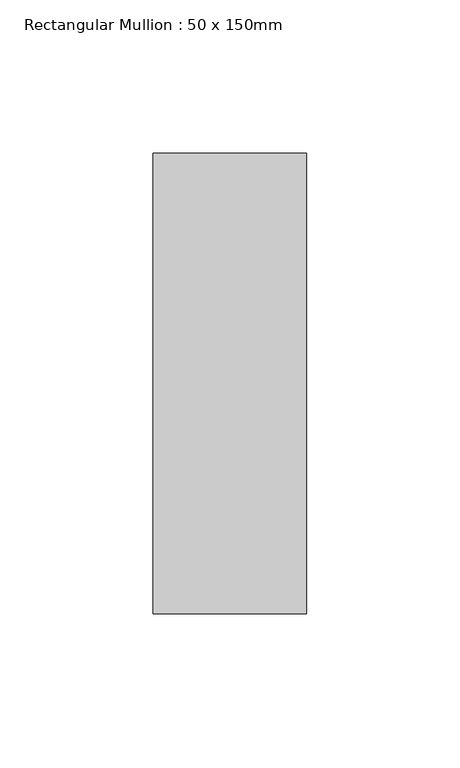
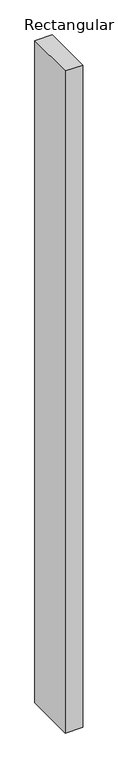
"""IFC4 building model written with IfcOpenShell, lengths in millimetres: member geometry, Rectangular Mullion : 50 x 150mm."""

import ifcopenshell
import ifcopenshell.guid

model = None  # the IFC model being written
_history = None  # IfcOwnerHistory: only IFC2X3 demands one
_inside = {}  # id of a spatial element -> (the spatial element, [elements in it])
_under = {}  # id of a project, library or spatial element -> (it, [spatial elements below it])
_declared = {}  # id of a project -> (the project, [libraries it declares])
_typed = {}  # id of a type object -> (the type object, [elements of that type])
_made_of = {}  # id of a material, layer set ... -> (it, [elements and type objects made of it])


def new_model(schema):
    """Start an empty IFC model of exactly this schema.

    Asked for "IFC4X3", IfcOpenShell would pick the latest addendum, in which some entities
    have other attributes; the version numbers below select the first issue.
    IFC2X3 requires an IfcOwnerHistory on every rooted entity: one is made here for all.
    """
    global model, _history
    if schema == "IFC4X3":
        model = ifcopenshell.file(schema_version=(4, 3, 0, 0))
    else:
        model = ifcopenshell.file(schema=schema)
    _inside.clear()
    _under.clear()
    _declared.clear()
    _typed.clear()
    _made_of.clear()
    _history = None
    if model.schema == "IFC2X3":
        org = make("IfcOrganization", Name="unknown")
        user = make(
            "IfcPersonAndOrganization",
            ThePerson=make("IfcPerson", FamilyName="unknown"),
            TheOrganization=org,
        )
        app = make(
            "IfcApplication",
            ApplicationDeveloper=org,
            Version="unknown",
            ApplicationFullName="unknown",
            ApplicationIdentifier="unknown",
        )
        _history = make(
            "IfcOwnerHistory",
            OwningUser=user,
            OwningApplication=app,
            ChangeAction="ADDED",
            CreationDate=0,
        )
    return model


def make(cls, **values):
    """One entity of the class cls with the attributes given. An attribute that is None is left unset."""
    return model.create_entity(
        cls, **{name: value for name, value in values.items() if value is not None}
    )


def rooted(cls, **values):
    """An entity with a GlobalId (a new one), such as an element, a storey or a relation."""
    return make(cls, GlobalId=ifcopenshell.guid.new(), OwnerHistory=_history, **values)


def si_unit(unit_type, name, prefix=None):
    """IfcSIUnit, for example si_unit("LENGTHUNIT", "METRE", prefix="MILLI")."""
    return make("IfcSIUnit", UnitType=unit_type, Prefix=prefix, Name=name)


def assignment(units):
    """IfcUnitAssignment: the units of a project."""
    return None if units is None else make("IfcUnitAssignment", Units=units)


def point(xyz):
    """IfcCartesianPoint."""
    return None if xyz is None else make("IfcCartesianPoint", Coordinates=xyz)


def direction(xyz):
    """IfcDirection."""
    return None if xyz is None else make("IfcDirection", DirectionRatios=xyz)


def frame(location, z_axis=None, x_axis=None):
    """IfcAxis2Placement3D, a coordinate frame: its origin and axes. An axis left out is left unset."""
    return make(
        "IfcAxis2Placement3D",
        Location=point(location),
        Axis=direction(z_axis),
        RefDirection=direction(x_axis),
    )


def origin():
    """The frame at (0, 0, 0) with its axes left unset."""
    return frame((0.0, 0.0, 0.0))


def place(relative_to, where):
    """IfcLocalPlacement: puts the frame where relative to a parent placement (None: the world)."""
    return make(
        "IfcLocalPlacement", PlacementRelTo=relative_to, RelativePlacement=where
    )


def context(
    kind, dimensions, precision=None, world=None, true_north=None, identifier=None
):
    """IfcGeometricRepresentationContext, for example the 3D "Model" context."""
    return make(
        "IfcGeometricRepresentationContext",
        ContextIdentifier=identifier,
        ContextType=kind,
        CoordinateSpaceDimension=dimensions,
        Precision=precision,
        WorldCoordinateSystem=world,
        TrueNorth=true_north,
    )


def project(units=None, contexts=None):
    """IfcProject with its units and contexts."""
    return rooted(
        "IfcProject",
        Name="project",
        RepresentationContexts=contexts,
        UnitsInContext=assignment(units),
    )


def spatial(cls, under=None, at=None, **own):
    """A site, building, storey or space (cls), placed at a placement, below another one or the project."""
    s = rooted(cls, ObjectPlacement=at, **own)
    if under is not None:
        _under.setdefault(under.id(), (under, []))[1].append(s)
    return s


def polyline(points):
    """IfcPolyline through the points."""
    return make("IfcPolyline", Points=[point(p) for p in points])


def outline(outer, holes=None, kind="AREA"):
    """IfcArbitraryClosedProfileDef: a profile drawn as a closed curve; with holes, ...WithVoids."""
    if holes is None:
        return make("IfcArbitraryClosedProfileDef", ProfileType=kind, OuterCurve=outer)
    return make(
        "IfcArbitraryProfileDefWithVoids",
        ProfileType=kind,
        OuterCurve=outer,
        InnerCurves=holes,
    )


def extrude(swept, where, along, depth):
    """IfcExtrudedAreaSolid: the profile swept, set in the frame where, extruded along a direction by depth."""
    return make(
        "IfcExtrudedAreaSolid",
        SweptArea=swept,
        Position=where,
        ExtrudedDirection=direction(along),
        Depth=depth,
    )


def shape(context_of_items, identifier, shape_type, items):
    """IfcShapeRepresentation: the items that make up one representation, for example the "Body"."""
    return make(
        "IfcShapeRepresentation",
        ContextOfItems=context_of_items,
        RepresentationIdentifier=identifier,
        RepresentationType=shape_type,
        Items=items,
    )


def source(mapping_origin, context_of_items, identifier, shape_type, items):
    """IfcRepresentationMap: a shape defined once, which mapped items show again and again."""
    return make(
        "IfcRepresentationMap",
        MappingOrigin=mapping_origin,
        MappedRepresentation=shape(context_of_items, identifier, shape_type, items),
    )


def transform(
    local_origin,
    x_axis=None,
    y_axis=None,
    z_axis=None,
    scale=None,
    scale2=None,
    scale3=None,
    uniform=True,
):
    """IfcCartesianTransformationOperator3D, or its non-uniform kind. x_axis, y_axis, z_axis: its Axis1, 2, 3."""
    if uniform:
        return make(
            "IfcCartesianTransformationOperator3D",
            Axis1=direction(x_axis),
            Axis2=direction(y_axis),
            LocalOrigin=point(local_origin),
            Scale=scale,
            Axis3=direction(z_axis),
        )
    return make(
        "IfcCartesianTransformationOperator3DnonUniform",
        Axis1=direction(x_axis),
        Axis2=direction(y_axis),
        LocalOrigin=point(local_origin),
        Scale=scale,
        Axis3=direction(z_axis),
        Scale2=scale2,
        Scale3=scale3,
    )


def mapped(mapping_source, mapping_target):
    """IfcMappedItem: shows the shape of a source again, moved by a transform."""
    return make(
        "IfcMappedItem", MappingSource=mapping_source, MappingTarget=mapping_target
    )


def made_of(thing, what):
    """Note that an element or type object is made of a material, layer set ...; save() writes the relation."""
    if what is not None:
        _made_of.setdefault(what.id(), (what, []))[1].append(thing)
    return thing


def element(
    cls,
    number,
    at=None,
    inside=None,
    cuts=None,
    type_object=None,
    material=None,
    context=None,
    identifier="Body",
    shape_type=None,
    held_by="IfcProductDefinitionShape",
    body=None,
    shapes=None,
    **own,
):
    """One element of the class cls, such as IfcWall. Its Tag is "e" and its number.

    at: its placement. inside: the storey or other place that contains it. cuts: it is an
    opening in that element (IfcRelVoidsElement). A single representation is given by context,
    identifier, shape_type and body (its items); several are given by shapes. held_by: the class
    of the entity that holds the representations. save() writes the other relations.
    """
    e = rooted(cls, Tag="e%d" % number, ObjectPlacement=at, **own)
    if body is not None:
        shapes = [shape(context, identifier, shape_type, body)]
    if shapes is not None:
        e.Representation = make(held_by, Representations=shapes)
    if inside is not None:
        _inside.setdefault(inside.id(), (inside, []))[1].append(e)
    if cuts is not None:
        rooted(
            "IfcRelVoidsElement", RelatingBuildingElement=cuts, RelatedOpeningElement=e
        )
    if type_object is not None:
        _typed.setdefault(type_object.id(), (type_object, []))[1].append(e)
    return made_of(e, material)


def aggregate(whole, parts):
    """IfcRelAggregates: a whole, such as a stair, and the parts it consists of."""
    return rooted("IfcRelAggregates", RelatingObject=whole, RelatedObjects=parts)


def save(model, path):
    """Write the relations noted so far, then the file.

    IfcRelAggregates (storeys below a building ...), IfcRelContainedInSpatialStructure (elements
    in a storey), IfcRelDefinesByType, IfcRelAssociatesMaterial and IfcRelDeclares: one each for
    every whole, place, type object, material and project.
    """
    for whole, parts in _under.values():
        aggregate(whole, parts)
    for where, things in _inside.values():
        rooted(
            "IfcRelContainedInSpatialStructure",
            RelatedElements=things,
            RelatingStructure=where,
        )
    for kind, things in _typed.values():
        rooted("IfcRelDefinesByType", RelatedObjects=things, RelatingType=kind)
    for what, things in _made_of.values():
        rooted("IfcRelAssociatesMaterial", RelatedObjects=things, RelatingMaterial=what)
    for by, libraries in _declared.values():
        rooted("IfcRelDeclares", RelatingContext=by, RelatedDefinitions=libraries)
    model.write(path)


def rectangular_mullion_50_x_150mm_3a148f0f(model_context):
    return source(origin(), model_context, "Body", "SweptSolid", [
        extrude(outline(polyline([(25.0, 75.0), (25.0, -75.0), (-25.0, -75.0), (-25.0, 75.0), (25.0, 75.0)])), frame((0.0, 0.0, -2000.0), z_axis=(0.0, 0.0, 1.0), x_axis=(1.0, 0.0, 0.0)), (0.0, 0.0, 1.0), 2000.0),
    ])


if __name__ == "__main__":
    model = new_model("IFC4")
    model_context = context("Model", 3, world=origin())
    ifc_project = project(units=[si_unit("LENGTHUNIT", "METRE", prefix="MILLI")], contexts=[model_context])
    site = spatial("IfcSite", under=ifc_project)
    building = spatial("IfcBuilding", under=site)
    placement = place(None, origin())
    rectangular_mullion_50_x_150mm_shape = rectangular_mullion_50_x_150mm_3a148f0f(model_context)
    element("IfcMember", 1, ObjectType="Rectangular Mullion : 50 x 150mm", at=placement, inside=building, context=model_context, shape_type="MappedRepresentation", body=[
        mapped(rectangular_mullion_50_x_150mm_shape, transform((0.0, 0.0, 0.0), x_axis=(1.0, 0.0, 0.0), y_axis=(0.0, 1.0, 0.0), z_axis=(0.0, 0.0, 1.0))),
    ])
    save(model, "model.ifc")

# Revit data of these elements
# Type "Rectangular Mullion : 50 x 150mm"
#   built-in parameter 1007304 = 0.492126 (stored number, unit not read)
#   built-in parameter 1007301 = 0.082021 (stored number, unit not read)
#   built-in parameter 1007300 = 0.082021 (stored number, unit not read)
# Element 1 (IfcMember, "Rectangular Mullion : 50 x 150mm")
#   Materials on its faces: "Metal - Aluminium"
# Materials
#   "Metal - Aluminium": class "Metal", colour RGB 247 247 247, transparency 0
